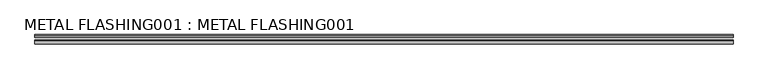
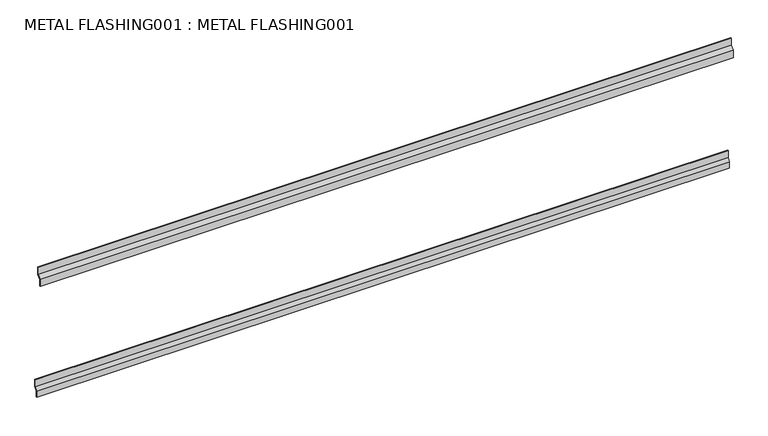
"""IFC4 building model written with IfcOpenShell, lengths in millimetres: proxy geometry, METAL FLASHING001 : METAL FLASHING001."""

from ifc_helpers import new_model, si_unit, frame, origin, place, context, project, spatial, polyline, outline, extrude, source, transform, mapped, element, save


def metal_flashing001_metal_flashing001_148fdf84(model_context):
    return source(origin(), model_context, "Body", "SweptSolid", [
        extrude(outline(polyline([(-5601.520996, 42709.570312), (-5611.268555, 42700.125), (-5611.268555, 42679.632812), (-5613.808555, 42679.632812), (-5613.808555, 42701.2006089), (-5604.060996, 42710.6459209), (-5604.060996, 42732.367188), (-5601.520996, 42732.367188), (-5601.520996, 42709.570312)])), frame((12382.7678845, 0.0, 0.0), z_axis=(1.0, 0.0, 0.0), x_axis=(0.0, 1.0, 0.0)), (0.0, 0.0, 1.0), 2000.25),
        extrude(outline(polyline([(-5586.8675368, 42358.078125), (-5592.980957, 42348.316406), (-5592.980957, 42330.03125), (-5595.520957, 42330.03125), (-5595.520957, 42349.0461179), (-5589.4075368, 42358.8078369), (-5589.4075368, 42380.582031), (-5586.8675368, 42380.582031), (-5586.8675368, 42358.078125)])), frame((12382.7678845, 0.0, 0.0), z_axis=(1.0, 0.0, 0.0), x_axis=(0.0, 1.0, 0.0)), (0.0, 0.0, 1.0), 2000.25),
    ])


if __name__ == "__main__":
    model = new_model("IFC4")
    model_context = context("Model", 3, world=origin())
    ifc_project = project(units=[si_unit("LENGTHUNIT", "METRE", prefix="MILLI")], contexts=[model_context])
    site = spatial("IfcSite", under=ifc_project)
    building = spatial("IfcBuilding", under=site)
    placement = place(None, origin())
    metal_flashing001_metal_flashing001_shape = metal_flashing001_metal_flashing001_148fdf84(model_context)
    element("IfcBuildingElementProxy", 1, Name="METAL FLASHING001 : METAL FLASHING001", ObjectType="METAL FLASHING001 : METAL FLASHING001", at=placement, inside=building, context=model_context, shape_type="MappedRepresentation", body=[
        mapped(metal_flashing001_metal_flashing001_shape, transform((0.0, 0.0, 0.0), x_axis=(1.0, 0.0, 0.0), y_axis=(0.0, 1.0, 0.0), z_axis=(0.0, 0.0, 1.0))),
    ])
    save(model, "model.ifc")

# Revit data of these elements
# Type "METAL FLASHING001 : METAL FLASHING001"
#   NameOverride = "METAL FLASHING001"
# Element 1 (IfcBuildingElementProxy, "METAL FLASHING001 : METAL FLASHING001")
#   Materials on its faces: "16 GA. COPPER BRAKE METAL FLASHING"
# Materials
#   "16 GA. COPPER BRAKE METAL FLASHING": class "Unassigned", colour RGB 128 128 128, transparency 0
